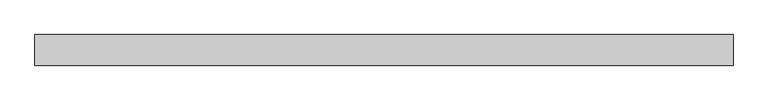
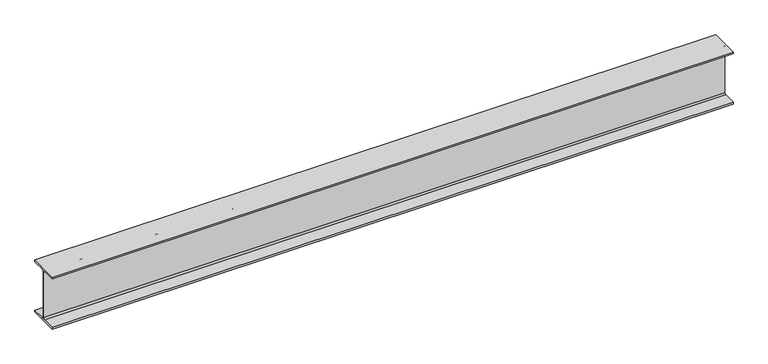
"""IFC4 building model written with IfcOpenShell, lengths in millimetres: beam geometry, Old_Steel Beam_H-KSD3502 : H_SB_ASB_H-200×200x8x12."""

import ifcopenshell
import ifcopenshell.guid

model = None  # the IFC model being written
_history = None  # IfcOwnerHistory: only IFC2X3 demands one
_inside = {}  # id of a spatial element -> (the spatial element, [elements in it])
_under = {}  # id of a project, library or spatial element -> (it, [spatial elements below it])
_declared = {}  # id of a project -> (the project, [libraries it declares])
_typed = {}  # id of a type object -> (the type object, [elements of that type])
_made_of = {}  # id of a material, layer set ... -> (it, [elements and type objects made of it])


def new_model(schema):
    """Start an empty IFC model of exactly this schema.

    Asked for "IFC4X3", IfcOpenShell would pick the latest addendum, in which some entities
    have other attributes; the version numbers below select the first issue.
    IFC2X3 requires an IfcOwnerHistory on every rooted entity: one is made here for all.
    """
    global model, _history
    if schema == "IFC4X3":
        model = ifcopenshell.file(schema_version=(4, 3, 0, 0))
    else:
        model = ifcopenshell.file(schema=schema)
    _inside.clear()
    _under.clear()
    _declared.clear()
    _typed.clear()
    _made_of.clear()
    _history = None
    if model.schema == "IFC2X3":
        org = make("IfcOrganization", Name="unknown")
        user = make(
            "IfcPersonAndOrganization",
            ThePerson=make("IfcPerson", FamilyName="unknown"),
            TheOrganization=org,
        )
        app = make(
            "IfcApplication",
            ApplicationDeveloper=org,
            Version="unknown",
            ApplicationFullName="unknown",
            ApplicationIdentifier="unknown",
        )
        _history = make(
            "IfcOwnerHistory",
            OwningUser=user,
            OwningApplication=app,
            ChangeAction="ADDED",
            CreationDate=0,
        )
    return model


def make(cls, **values):
    """One entity of the class cls with the attributes given. An attribute that is None is left unset."""
    return model.create_entity(
        cls, **{name: value for name, value in values.items() if value is not None}
    )


def rooted(cls, **values):
    """An entity with a GlobalId (a new one), such as an element, a storey or a relation."""
    return make(cls, GlobalId=ifcopenshell.guid.new(), OwnerHistory=_history, **values)


def si_unit(unit_type, name, prefix=None):
    """IfcSIUnit, for example si_unit("LENGTHUNIT", "METRE", prefix="MILLI")."""
    return make("IfcSIUnit", UnitType=unit_type, Prefix=prefix, Name=name)


def assignment(units):
    """IfcUnitAssignment: the units of a project."""
    return None if units is None else make("IfcUnitAssignment", Units=units)


def point(xyz):
    """IfcCartesianPoint."""
    return None if xyz is None else make("IfcCartesianPoint", Coordinates=xyz)


def direction(xyz):
    """IfcDirection."""
    return None if xyz is None else make("IfcDirection", DirectionRatios=xyz)


def frame(location, z_axis=None, x_axis=None):
    """IfcAxis2Placement3D, a coordinate frame: its origin and axes. An axis left out is left unset."""
    return make(
        "IfcAxis2Placement3D",
        Location=point(location),
        Axis=direction(z_axis),
        RefDirection=direction(x_axis),
    )


def frame_2d(location, x_axis=None):
    """IfcAxis2Placement2D, a coordinate frame in the plane: its origin and x axis."""
    return make(
        "IfcAxis2Placement2D", Location=point(location), RefDirection=direction(x_axis)
    )


def origin():
    """The frame at (0, 0, 0) with its axes left unset."""
    return frame((0.0, 0.0, 0.0))


def place(relative_to, where):
    """IfcLocalPlacement: puts the frame where relative to a parent placement (None: the world)."""
    return make(
        "IfcLocalPlacement", PlacementRelTo=relative_to, RelativePlacement=where
    )


def context(
    kind, dimensions, precision=None, world=None, true_north=None, identifier=None
):
    """IfcGeometricRepresentationContext, for example the 3D "Model" context."""
    return make(
        "IfcGeometricRepresentationContext",
        ContextIdentifier=identifier,
        ContextType=kind,
        CoordinateSpaceDimension=dimensions,
        Precision=precision,
        WorldCoordinateSystem=world,
        TrueNorth=true_north,
    )


def project(units=None, contexts=None):
    """IfcProject with its units and contexts."""
    return rooted(
        "IfcProject",
        Name="project",
        RepresentationContexts=contexts,
        UnitsInContext=assignment(units),
    )


def spatial(cls, under=None, at=None, **own):
    """A site, building, storey or space (cls), placed at a placement, below another one or the project."""
    s = rooted(cls, ObjectPlacement=at, **own)
    if under is not None:
        _under.setdefault(under.id(), (under, []))[1].append(s)
    return s


def polyline(points):
    """IfcPolyline through the points."""
    return make("IfcPolyline", Points=[point(p) for p in points])


def circle_curve(where, radius):
    """IfcCircle in the frame where."""
    return make("IfcCircle", Position=where, Radius=radius)


def trimmed(basis, trim1, trim2, sense, master):
    """IfcTrimmedCurve: the piece of a basis curve between two trims."""
    return make(
        "IfcTrimmedCurve",
        BasisCurve=basis,
        Trim1=trim1,
        Trim2=trim2,
        SenseAgreement=sense,
        MasterRepresentation=master,
    )


def segment(curve, same_sense, transition):
    """IfcCompositeCurveSegment."""
    return make(
        "IfcCompositeCurveSegment",
        Transition=transition,
        SameSense=same_sense,
        ParentCurve=curve,
    )


def composite_curve(segments, self_intersect=None):
    """IfcCompositeCurve: segments joined end to end."""
    return make("IfcCompositeCurve", Segments=segments, SelfIntersect=self_intersect)


def outline(outer, holes=None, kind="AREA"):
    """IfcArbitraryClosedProfileDef: a profile drawn as a closed curve; with holes, ...WithVoids."""
    if holes is None:
        return make("IfcArbitraryClosedProfileDef", ProfileType=kind, OuterCurve=outer)
    return make(
        "IfcArbitraryProfileDefWithVoids",
        ProfileType=kind,
        OuterCurve=outer,
        InnerCurves=holes,
    )


def extrude(swept, where, along, depth):
    """IfcExtrudedAreaSolid: the profile swept, set in the frame where, extruded along a direction by depth."""
    return make(
        "IfcExtrudedAreaSolid",
        SweptArea=swept,
        Position=where,
        ExtrudedDirection=direction(along),
        Depth=depth,
    )


def shape(context_of_items, identifier, shape_type, items):
    """IfcShapeRepresentation: the items that make up one representation, for example the "Body"."""
    return make(
        "IfcShapeRepresentation",
        ContextOfItems=context_of_items,
        RepresentationIdentifier=identifier,
        RepresentationType=shape_type,
        Items=items,
    )


def source(mapping_origin, context_of_items, identifier, shape_type, items):
    """IfcRepresentationMap: a shape defined once, which mapped items show again and again."""
    return make(
        "IfcRepresentationMap",
        MappingOrigin=mapping_origin,
        MappedRepresentation=shape(context_of_items, identifier, shape_type, items),
    )


def transform(
    local_origin,
    x_axis=None,
    y_axis=None,
    z_axis=None,
    scale=None,
    scale2=None,
    scale3=None,
    uniform=True,
):
    """IfcCartesianTransformationOperator3D, or its non-uniform kind. x_axis, y_axis, z_axis: its Axis1, 2, 3."""
    if uniform:
        return make(
            "IfcCartesianTransformationOperator3D",
            Axis1=direction(x_axis),
            Axis2=direction(y_axis),
            LocalOrigin=point(local_origin),
            Scale=scale,
            Axis3=direction(z_axis),
        )
    return make(
        "IfcCartesianTransformationOperator3DnonUniform",
        Axis1=direction(x_axis),
        Axis2=direction(y_axis),
        LocalOrigin=point(local_origin),
        Scale=scale,
        Axis3=direction(z_axis),
        Scale2=scale2,
        Scale3=scale3,
    )


def mapped(mapping_source, mapping_target):
    """IfcMappedItem: shows the shape of a source again, moved by a transform."""
    return make(
        "IfcMappedItem", MappingSource=mapping_source, MappingTarget=mapping_target
    )


def made_of(thing, what):
    """Note that an element or type object is made of a material, layer set ...; save() writes the relation."""
    if what is not None:
        _made_of.setdefault(what.id(), (what, []))[1].append(thing)
    return thing


def element(
    cls,
    number,
    at=None,
    inside=None,
    cuts=None,
    type_object=None,
    material=None,
    context=None,
    identifier="Body",
    shape_type=None,
    held_by="IfcProductDefinitionShape",
    body=None,
    shapes=None,
    **own,
):
    """One element of the class cls, such as IfcWall. Its Tag is "e" and its number.

    at: its placement. inside: the storey or other place that contains it. cuts: it is an
    opening in that element (IfcRelVoidsElement). A single representation is given by context,
    identifier, shape_type and body (its items); several are given by shapes. held_by: the class
    of the entity that holds the representations. save() writes the other relations.
    """
    e = rooted(cls, Tag="e%d" % number, ObjectPlacement=at, **own)
    if body is not None:
        shapes = [shape(context, identifier, shape_type, body)]
    if shapes is not None:
        e.Representation = make(held_by, Representations=shapes)
    if inside is not None:
        _inside.setdefault(inside.id(), (inside, []))[1].append(e)
    if cuts is not None:
        rooted(
            "IfcRelVoidsElement", RelatingBuildingElement=cuts, RelatedOpeningElement=e
        )
    if type_object is not None:
        _typed.setdefault(type_object.id(), (type_object, []))[1].append(e)
    return made_of(e, material)


def aggregate(whole, parts):
    """IfcRelAggregates: a whole, such as a stair, and the parts it consists of."""
    return rooted("IfcRelAggregates", RelatingObject=whole, RelatedObjects=parts)


def save(model, path):
    """Write the relations noted so far, then the file.

    IfcRelAggregates (storeys below a building ...), IfcRelContainedInSpatialStructure (elements
    in a storey), IfcRelDefinesByType, IfcRelAssociatesMaterial and IfcRelDeclares: one each for
    every whole, place, type object, material and project.
    """
    for whole, parts in _under.values():
        aggregate(whole, parts)
    for where, things in _inside.values():
        rooted(
            "IfcRelContainedInSpatialStructure",
            RelatedElements=things,
            RelatingStructure=where,
        )
    for kind, things in _typed.values():
        rooted("IfcRelDefinesByType", RelatedObjects=things, RelatingType=kind)
    for what, things in _made_of.values():
        rooted("IfcRelAssociatesMaterial", RelatedObjects=things, RelatingMaterial=what)
    for by, libraries in _declared.values():
        rooted("IfcRelDeclares", RelatingContext=by, RelatedDefinitions=libraries)
    model.write(path)


def beam_cb92c45f(model_context):
    return source(origin(), model_context, "Body", "SweptSolid", [
        extrude(outline(composite_curve([segment(polyline([(82.5, -141.5), (82.5, -151.7), (-82.5, -151.7), (-82.5, -141.5), (-11.9, -141.5)]), True, "CONTINUOUS"), segment(trimmed(circle_curve(frame_2d((-11.9, -132.6)), 8.9), [point((-11.9, -141.5))], [point((-3.0, -132.6))], True, "CARTESIAN"), True, "CONTINUOUS"), segment(polyline([(-3.0, -132.6), (-3.0, 132.6)]), True, "CONTINUOUS"), segment(trimmed(circle_curve(frame_2d((-11.9, 132.6)), 8.9), [point((-3.0, 132.6))], [point((-11.9, 141.5))], True, "CARTESIAN"), True, "CONTINUOUS"), segment(polyline([(-11.9, 141.5), (-82.5, 141.5), (-82.5, 151.7), (82.5, 151.7), (82.5, 141.5), (11.9, 141.5)]), True, "CONTINUOUS"), segment(trimmed(circle_curve(frame_2d((11.9, 132.6)), 8.9), [point((11.9, 141.5))], [point((3.0, 132.6))], True, "CARTESIAN"), True, "CONTINUOUS"), segment(polyline([(3.0, 132.6), (3.0, -132.6)]), True, "CONTINUOUS"), segment(trimmed(circle_curve(frame_2d((11.9, -132.6)), 8.9), [point((3.0, -132.6))], [point((11.9, -141.5))], True, "CARTESIAN"), True, "CONTINUOUS"), segment(polyline([(11.9, -141.5), (82.5, -141.5)]), True, "CONTINUOUS")], self_intersect=False)), frame((-1938.4214468, 0.0, 0.0), z_axis=(1.0, 0.0, 0.0), x_axis=(0.0, 1.0, 0.0)), (0.0, 0.0, 1.0), 3758.8913358),
    ])


if __name__ == "__main__":
    model = new_model("IFC4")
    model_context = context("Model", 3, world=origin())
    ifc_project = project(units=[si_unit("LENGTHUNIT", "METRE", prefix="MILLI")], contexts=[model_context])
    site = spatial("IfcSite", under=ifc_project)
    building = spatial("IfcBuilding", under=site)
    placement = place(None, origin())
    beam_shape = beam_cb92c45f(model_context)
    element("IfcBeam", 1, ObjectType="Old_Steel Beam_H-KSD3502 : H_SB_ASB_H-200×200x8x12", at=placement, inside=building, context=model_context, shape_type="MappedRepresentation", body=[
        mapped(beam_shape, transform((0.0, 0.0, 0.0), x_axis=(1.0, 0.0, 0.0), y_axis=(0.0, 1.0, 0.0), z_axis=(0.0, 0.0, 1.0))),
    ])
    save(model, "model.ifc")

# Revit data of these elements
# Type "Old_Steel Beam_H-KSD3502 : H_SB_ASB_H-200×200x8x12"
#   Width = 20.0 cm
#   Web Thickness = 0.8 cm
#   Web Fillet = 1.3 cm
#   Warping Constant = 141376.0 cm⁶
#   Torsional Moment of Inertia = 26.2485 cm⁴
#   Torsional Modulus = 1.0 cm³
#   Section Area = 63.53 cm²
#   Plastic Modulus weak axis = 244.0 cm³
#   Plastic Modulus strong axis = 525.0 cm³
#   Perimeter = 1.16 m²/m
#   Nominal Weight = 49.90 kgf/m
#   Moment of Inertia weak axis = 1600.00 cm⁴
#   Moment of Inertia strong axis = 4720.00 cm⁴
#   Height = 20.0 cm
#   Flange Thickness = 1.2 cm
#   Elastic Modulus weak axis = 160.0 cm³
#   Elastic Modulus strong axis = 472.0 cm³
#   Centroid Vertical = 10.0 cm
#   Centroid Horizontal = 10.0 cm
#   Length [instance default] = 1.5240 m
#   Structural Material [instance default] = Steel, 45-345
#   Assembly Code = ""
# Element 1 (IfcBeam, "Old_Steel Beam_H-KSD3502 : H_SB_ASB_H-200×200x8x12")
#   Structural Material = none
# Materials
#   "Steel, 45-345": class "Metal", colour RGB 189 187 185, transparency 0, Description = "Steel 345 MPa", Cost = 0
